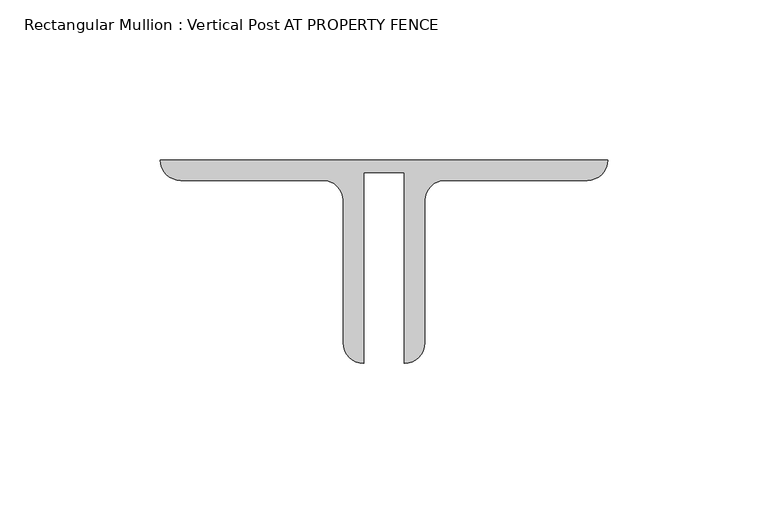
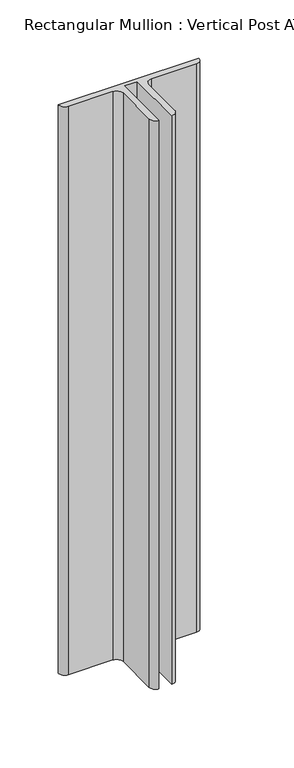
"""IFC4 building model written with IfcOpenShell, lengths in millimetres: member geometry, Rectangular Mullion : Vertical Post AT PROPERTY FENCE."""

from ifc_helpers import new_model, si_unit, point, frame, frame_2d, origin, place, context, project, spatial, polyline, circle_curve, trimmed, segment, composite_curve, outline, extrude, source, transform, mapped, element, save


def rectangular_mullion_vertical_post_at_property_fence_e70192c4(model_context):
    return source(origin(), model_context, "Body", "SweptSolid", [
        extrude(outline(composite_curve([segment(polyline([(-63.5, -22.9145205), (-76.2, -22.9145205), (-76.2, -82.55)]), True, "CONTINUOUS"), segment(trimmed(circle_curve(frame_2d((-76.2, -76.2)), 6.35), [point((-76.2, -82.55))], [point((-82.55, -76.2))], False, "CARTESIAN"), True, "CONTINUOUS"), segment(polyline([(-82.55, -76.2), (-82.55, -31.75)]), True, "CONTINUOUS"), segment(trimmed(circle_curve(frame_2d((-88.9, -31.75)), 6.35), [point((-82.55, -31.75))], [point((-88.9, -25.4))], True, "CARTESIAN"), True, "CONTINUOUS"), segment(polyline([(-88.9, -25.4), (-133.35, -25.4)]), True, "CONTINUOUS"), segment(trimmed(circle_curve(frame_2d((-133.35, -19.05)), 6.35), [point((-133.35, -25.4))], [point((-139.7, -19.05))], False, "CARTESIAN"), True, "CONTINUOUS"), segment(polyline([(-139.7, -19.05), (0.0, -19.05)]), True, "CONTINUOUS"), segment(trimmed(circle_curve(frame_2d((-6.35, -19.05)), 6.35), [point((0.0, -19.05))], [point((-6.35, -25.4))], False, "CARTESIAN"), True, "CONTINUOUS"), segment(polyline([(-6.35, -25.4), (-50.8, -25.4)]), True, "CONTINUOUS"), segment(trimmed(circle_curve(frame_2d((-50.8, -31.75)), 6.35), [point((-50.8, -25.4))], [point((-57.15, -31.75))], True, "CARTESIAN"), True, "CONTINUOUS"), segment(polyline([(-57.15, -31.75), (-57.15, -76.2)]), True, "CONTINUOUS"), segment(trimmed(circle_curve(frame_2d((-63.5, -76.2)), 6.35), [point((-57.15, -76.2))], [point((-63.5, -82.55))], False, "CARTESIAN"), True, "CONTINUOUS"), segment(polyline([(-63.5, -82.55), (-63.5, -22.9145205)]), True, "CONTINUOUS")], self_intersect=False)), frame((0.0, 0.0, -596.9), z_axis=(0.0, 0.0, 1.0), x_axis=(1.0, 0.0, 0.0)), (0.0, 0.0, 1.0), 596.9),
    ])


if __name__ == "__main__":
    model = new_model("IFC4")
    model_context = context("Model", 3, world=origin())
    ifc_project = project(units=[si_unit("LENGTHUNIT", "METRE", prefix="MILLI")], contexts=[model_context])
    site = spatial("IfcSite", under=ifc_project)
    building = spatial("IfcBuilding", under=site)
    placement = place(None, origin())
    rectangular_mullion_vertical_post_at_property_fence_shape = rectangular_mullion_vertical_post_at_property_fence_e70192c4(model_context)
    element("IfcMember", 1, ObjectType="Rectangular Mullion : Vertical Post AT PROPERTY FENCE", at=placement, inside=building, context=model_context, shape_type="MappedRepresentation", body=[
        mapped(rectangular_mullion_vertical_post_at_property_fence_shape, transform((0.0, 0.0, 0.0), x_axis=(1.0, 0.0, 0.0), y_axis=(0.0, 1.0, 0.0), z_axis=(0.0, 0.0, 1.0))),
    ])
    save(model, "model.ifc")

# Revit data of these elements
# Type "Rectangular Mullion : Vertical Post AT PROPERTY FENCE"
#   built-in parameter 1007351 = -0.0625 (stored number, unit not read)
#   built-in parameter 1007322 = 0.0126789 (stored number, unit not read)
#   built-in parameter 1007321 = 0.229167 (stored number, unit not read)
#   built-in parameter 1007320 = 0.229167 (stored number, unit not read)
# Element 1 (IfcMember, "Rectangular Mullion : Vertical Post AT PROPERTY FENCE")
#   Materials on its faces: "MAIN FENCE POST: (2) BACK/BACK GALVANIZED ANGLES (2) L2 1/2 X 2 1/2 X 1/4\") ANCHORED TO 8\"W X 42\" DEEP CONCRETE FOOTING(1)"
# Materials
#   "MAIN FENCE POST: (2) BACK/BACK GALVANIZED ANGLES (2) L2 1/2 X 2 1/2 X 1/4\") ANCHORED TO 8\"W X 42\" DEEP CONCRETE FOOTING(1)": class "Unassigned", colour RGB 211 211 211, transparency 0, Cost = 0
